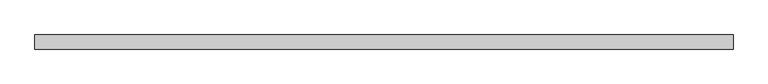
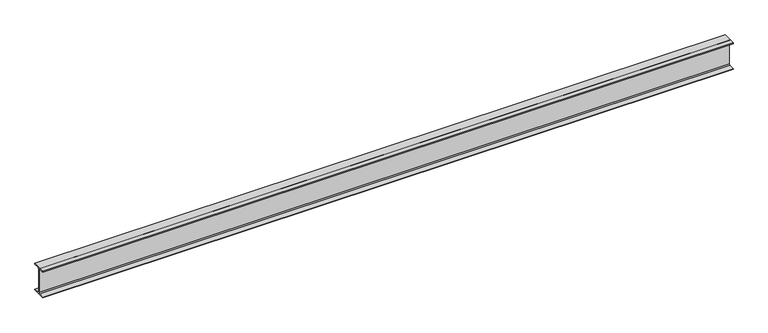
"""IFC4 building model written with IfcOpenShell, lengths in millimetres: beam geometry, 0912_Steel Framing_H-KSD3502 : H_SB_ASB_H-350x175x7x11."""

from ifc_helpers import new_model, si_unit, point, frame, frame_2d, origin, place, context, project, spatial, polyline, circle_curve, trimmed, segment, composite_curve, outline, extrude, source, transform, mapped, element, save


def beam_8f1eb5a0(model_context):
    return source(origin(), model_context, "Body", "SweptSolid", [
        extrude(outline(composite_curve([segment(polyline([(87.5, -164.0), (87.5, -175.0), (-87.5, -175.0), (-87.5, -164.0), (-17.5, -164.0)]), True, "CONTINUOUS"), segment(trimmed(circle_curve(frame_2d((-17.5, -150.0)), 14.0), [point((-17.5, -164.0))], [point((-3.5, -150.0))], True, "CARTESIAN"), True, "CONTINUOUS"), segment(polyline([(-3.5, -150.0), (-3.5, 150.0)]), True, "CONTINUOUS"), segment(trimmed(circle_curve(frame_2d((-17.5, 150.0)), 14.0), [point((-3.5, 150.0))], [point((-17.5, 164.0))], True, "CARTESIAN"), True, "CONTINUOUS"), segment(polyline([(-17.5, 164.0), (-87.5, 164.0), (-87.5, 175.0), (87.5, 175.0), (87.5, 164.0), (17.5, 164.0)]), True, "CONTINUOUS"), segment(trimmed(circle_curve(frame_2d((17.5, 150.0)), 14.0), [point((17.5, 164.0))], [point((3.5, 150.0))], True, "CARTESIAN"), True, "CONTINUOUS"), segment(polyline([(3.5, 150.0), (3.5, -150.0)]), True, "CONTINUOUS"), segment(trimmed(circle_curve(frame_2d((17.5, -150.0)), 14.0), [point((3.5, -150.0))], [point((17.5, -164.0))], True, "CARTESIAN"), True, "CONTINUOUS"), segment(polyline([(17.5, -164.0), (87.5, -164.0)]), True, "CONTINUOUS")], self_intersect=False)), frame((-4333.8712061, 0.0, 0.0), z_axis=(1.0, 0.0, 0.0), x_axis=(0.0, 1.0, 0.0)), (0.0, 0.0, 1.0), 8632.7424123),
    ])


if __name__ == "__main__":
    model = new_model("IFC4")
    model_context = context("Model", 3, world=origin())
    ifc_project = project(units=[si_unit("LENGTHUNIT", "METRE", prefix="MILLI")], contexts=[model_context])
    site = spatial("IfcSite", under=ifc_project)
    building = spatial("IfcBuilding", under=site)
    placement = place(None, origin())
    beam_shape = beam_8f1eb5a0(model_context)
    element("IfcBeam", 1, ObjectType="0912_Steel Framing_H-KSD3502 : H_SB_ASB_H-350x175x7x11", at=placement, inside=building, context=model_context, shape_type="MappedRepresentation", body=[
        mapped(beam_shape, transform((0.0, 0.0, 0.0), x_axis=(1.0, 0.0, 0.0), y_axis=(0.0, 1.0, 0.0), z_axis=(0.0, 0.0, 1.0))),
    ])
    save(model, "model.ifc")

# Revit data of these elements
# Type "0912_Steel Framing_H-KSD3502 : H_SB_ASB_H-350x175x7x11"
#   H_WM Code_1 = "S01AA002-00001 | Main Steel Structure Fabrication Work | Shelter/Building | Medium Steel - Standard (90KG/M>Weight≥30KG/M) | Material: (   )"
#   H_WM Code_2 = "S03AA028-00001 | Main Steel Structure Erection Work | Shelter/Building | Medium Steel (90KG/M>Weight≥30KG/M) | Material: (   )"
#   H_WM Code_3 = "S01AA010-00001 | Main Steel Structure Fabrication Work | Shelter/Building | Steel Painting/Coating | for Non-Fireproofed Steel Surface, Surface Preparation, Primer, Second & Final Coat | Material: (   )"
#   H_Q'ty Cal Type Tag = "SB-Q2"
#   Width = 17.5 cm
#   Web Thickness = 0.7 cm
#   Web Fillet = 1.4 cm
#   Warping Constant = 282000.0 cm⁶
#   W = 0
#   Torsional Moment of Inertia = 19.4042 cm⁴
#   Section Area = 63.14 cm²
#   Plastic Modulus weak axis = 174.0 cm³
#   Plastic Modulus strong axis = 868.0 cm³
#   Perimeter = 1.36 m²/m
#   Nominal Weight = 49.60 kgf/m
#   Moment of Inertia weak axis = 984.00 cm⁴
#   Moment of Inertia strong axis = 13600.00 cm⁴
#   Height = 35.0 cm
#   Flange Thickness = 1.1 cm
#   Elastic Modulus weak axis = 112.0 cm³
#   Elastic Modulus strong axis = 775.0 cm³
#   Centroid Vertical = 17.5 cm
#   Centroid Horizontal = 8.75 cm
#   Ix = 136000000
#   Length [instance default] = 1.5240 m
#   Zx = 868000
#   b = 0.1750 m
#   h = 0.3500 m
#   r = 0.0140 m
#   s = 0.0070 m
#   t = 0.0110 m
#   A = 0.006314 m²
#   Structural Material [instance default] = Steel, 45-345
#   Assembly Code = ""
# Element 1 (IfcBeam, "0912_Steel Framing_H-KSD3502 : H_SB_ASB_H-350x175x7x11")
#   Structural Material = none
# Materials
#   "Steel, 45-345": class "Metal", colour RGB 189 187 185, transparency 0, Description = "Steel 345 MPa", Cost = 0
